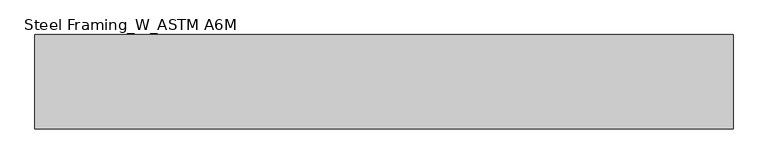
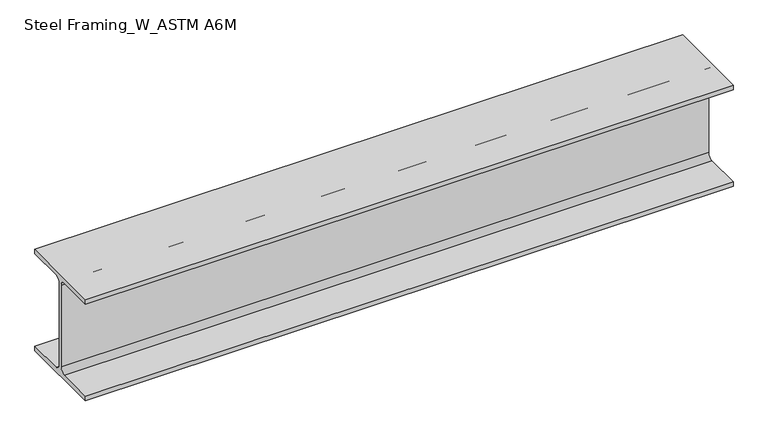
"""IFC4 building model written with IfcOpenShell, lengths in millimetres: beam geometry, Steel Framing_W_ASTM A6M : H_SB_AR_S02_W250x49.1_RCG1."""

from ifc_helpers import new_model, si_unit, point, frame, frame_2d, origin, place, context, project, spatial, polyline, circle_curve, trimmed, segment, composite_curve, outline, extrude, source, transform, mapped, element, save


def steel_framing_w_astm_a6m_ab5abfa9(model_context):
    return source(origin(), model_context, "Body", "SweptSolid", [
        extrude(outline(composite_curve([segment(polyline([(101.0, -112.5), (101.0, -123.5), (-101.0, -123.5), (-101.0, -112.5), (-16.385, -112.5)]), True, "CONTINUOUS"), segment(trimmed(circle_curve(frame_2d((-16.385, -99.8)), 12.7), [point((-16.385, -112.5))], [point((-3.685, -99.8))], True, "CARTESIAN"), True, "CONTINUOUS"), segment(polyline([(-3.685, -99.8), (-3.685, 99.8)]), True, "CONTINUOUS"), segment(trimmed(circle_curve(frame_2d((-16.385, 99.8)), 12.7), [point((-3.685, 99.8))], [point((-16.385, 112.5))], True, "CARTESIAN"), True, "CONTINUOUS"), segment(polyline([(-16.385, 112.5), (-101.0, 112.5), (-101.0, 123.5), (101.0, 123.5), (101.0, 112.5), (16.385, 112.5)]), True, "CONTINUOUS"), segment(trimmed(circle_curve(frame_2d((16.385, 99.8)), 12.7), [point((16.385, 112.5))], [point((3.685, 99.8))], True, "CARTESIAN"), True, "CONTINUOUS"), segment(polyline([(3.685, 99.8), (3.685, -99.8)]), True, "CONTINUOUS"), segment(trimmed(circle_curve(frame_2d((16.385, -99.8)), 12.7), [point((3.685, -99.8))], [point((16.385, -112.5))], True, "CARTESIAN"), True, "CONTINUOUS"), segment(polyline([(16.385, -112.5), (101.0, -112.5)]), True, "CONTINUOUS")], self_intersect=False)), frame((-747.55, 0.0, 0.0), z_axis=(1.0, 0.0, 0.0), x_axis=(0.0, 1.0, 0.0)), (0.0, 0.0, 1.0), 1495.1),
    ])


if __name__ == "__main__":
    model = new_model("IFC4")
    model_context = context("Model", 3, world=origin())
    ifc_project = project(units=[si_unit("LENGTHUNIT", "METRE", prefix="MILLI")], contexts=[model_context])
    site = spatial("IfcSite", under=ifc_project)
    building = spatial("IfcBuilding", under=site)
    placement = place(None, origin())
    steel_framing_w_astm_a6m_shape = steel_framing_w_astm_a6m_ab5abfa9(model_context)
    element("IfcBeam", 1, ObjectType="Steel Framing_W_ASTM A6M : H_SB_AR_S02_W250x49.1_RCG1", at=placement, inside=building, context=model_context, shape_type="MappedRepresentation", body=[
        mapped(steel_framing_w_astm_a6m_shape, transform((0.0, 0.0, 0.0), x_axis=(1.0, 0.0, 0.0), y_axis=(0.0, 1.0, 0.0), z_axis=(0.0, 0.0, 1.0))),
    ])
    save(model, "model.ifc")

# Revit data of these elements
# Type "Steel Framing_W_ASTM A6M : H_SB_AR_S02_W250x49.1_RCG1"
#   Type Mark = "RCG1"
#   Section Name Key = "W10x33"
#   Width = 20.2 cm
#   Web Thickness = 0.737 cm
#   Web Fillet = 1.27 cm
#   Warping Constant = 212000.0 cm⁶
#   Torsional Moment of Inertia = 24.30 cm⁴
#   Section Area = 62.6 cm²
#   Plastic Modulus weak axis = 229.0 cm³
#   Plastic Modulus strong axis = 636.0 cm³
#   Perimeter = 1.27 m²/m
#   Nominal Weight = 49.10 kgf/m
#   Moment of Inertia weak axis = 1520.00 cm⁴
#   Moment of Inertia strong axis = 7120.00 cm⁴
#   Height = 24.7 cm
#   Flange Thickness = 1.1 cm
#   Elastic Modulus weak axis = 151.0 cm³
#   Elastic Modulus strong axis = 574.0 cm³
#   Centroid Vertical = 12.35 cm
#   Centroid Horizontal = 10.1 cm
#   Length [instance default] = 1500 mm
#   Structural Material [instance default] = Steel, 45-345
#   Bolt Spacing = 0
#   Assembly Code = ""
# Element 1 (IfcBeam, "Steel Framing_W_ASTM A6M : H_SB_AR_S02_W250x49.1_RCG1")
#   Materials on its faces: "Steel, 45-345"
# Materials
#   "Steel, 45-345": class "Metal", colour RGB 189 187 185, transparency 0, Description = "Steel 345 MPa", Cost = 0
